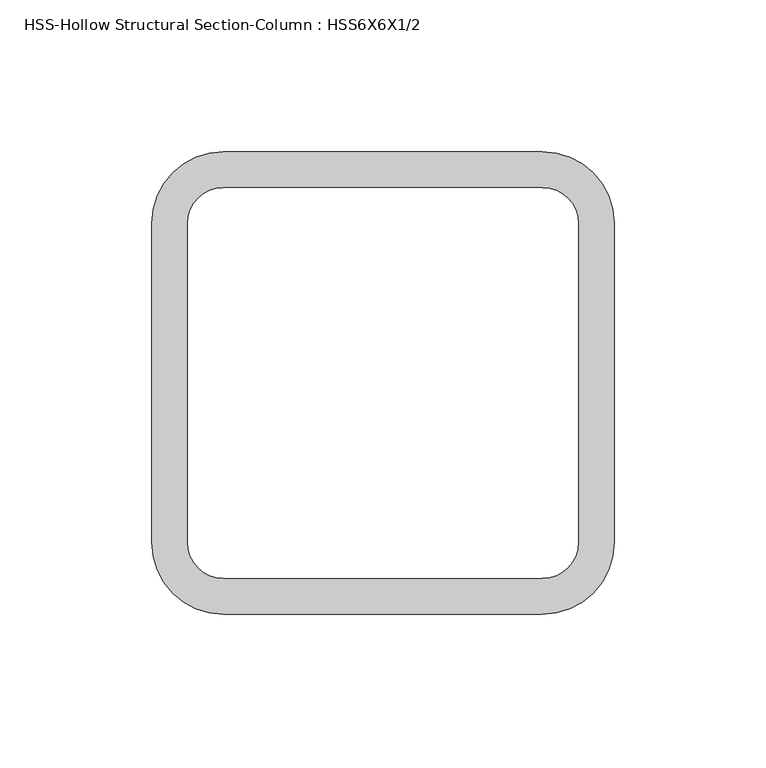
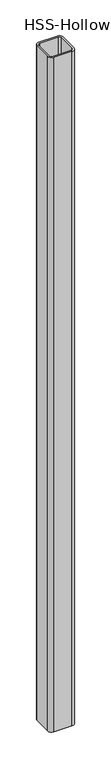
"""IFC4 building model written with IfcOpenShell, lengths in millimetres: column geometry, HSS-Hollow Structural Section-Column : HSS6X6X1/2."""

from ifc_helpers import new_model, si_unit, point, frame_2d, origin, origin_with_axes, place, context, project, spatial, polyline, circle_curve, trimmed, segment, composite_curve, outline, extrude, source, transform, mapped, element, save


def hss_hollow_structural_section_column_hss6x6x1_2_37f7f079(model_context):
    return source(origin(), model_context, "Body", "SweptSolid", [
        extrude(outline(composite_curve([segment(trimmed(circle_curve(frame_2d((52.578, 52.578)), 23.622), [point((52.578, 76.2))], [point((76.2, 52.578))], False, "CARTESIAN"), True, "CONTINUOUS"), segment(polyline([(76.2, 52.578), (76.2, -52.578)]), True, "CONTINUOUS"), segment(trimmed(circle_curve(frame_2d((52.578, -52.578)), 23.622), [point((76.2, -52.578))], [point((52.578, -76.2))], False, "CARTESIAN"), True, "CONTINUOUS"), segment(polyline([(52.578, -76.2), (-52.578, -76.2)]), True, "CONTINUOUS"), segment(trimmed(circle_curve(frame_2d((-52.578, -52.578)), 23.622), [point((-52.578, -76.2))], [point((-76.2, -52.578))], False, "CARTESIAN"), True, "CONTINUOUS"), segment(polyline([(-76.2, -52.578), (-76.2, 52.578)]), True, "CONTINUOUS"), segment(trimmed(circle_curve(frame_2d((-52.578, 52.578)), 23.622), [point((-76.2, 52.578))], [point((-52.578, 76.2))], False, "CARTESIAN"), True, "CONTINUOUS"), segment(polyline([(-52.578, 76.2), (52.578, 76.2)]), True, "CONTINUOUS")], self_intersect=False), holes=[composite_curve([segment(polyline([(52.578, 64.389), (-52.578, 64.389)]), True, "CONTINUOUS"), segment(trimmed(circle_curve(frame_2d((-52.578, 52.578)), 11.811), [point((-52.578, 64.389))], [point((-64.389, 52.578))], True, "CARTESIAN"), True, "CONTINUOUS"), segment(polyline([(-64.389, 52.578), (-64.389, -52.578)]), True, "CONTINUOUS"), segment(trimmed(circle_curve(frame_2d((-52.578, -52.578)), 11.811), [point((-64.389, -52.578))], [point((-52.578, -64.389))], True, "CARTESIAN"), True, "CONTINUOUS"), segment(polyline([(-52.578, -64.389), (52.578, -64.389)]), True, "CONTINUOUS"), segment(trimmed(circle_curve(frame_2d((52.578, -52.578)), 11.811), [point((52.578, -64.389))], [point((64.389, -52.578))], True, "CARTESIAN"), True, "CONTINUOUS"), segment(polyline([(64.389, -52.578), (64.389, 52.578)]), True, "CONTINUOUS"), segment(trimmed(circle_curve(frame_2d((52.578, 52.578)), 11.811), [point((64.389, 52.578))], [point((52.578, 64.389))], True, "CARTESIAN"), True, "CONTINUOUS")], self_intersect=False)]), origin_with_axes(), (0.0, 0.0, 1.0), 4127.5),
    ])


if __name__ == "__main__":
    model = new_model("IFC4")
    model_context = context("Model", 3, world=origin())
    ifc_project = project(units=[si_unit("LENGTHUNIT", "METRE", prefix="MILLI")], contexts=[model_context])
    site = spatial("IfcSite", under=ifc_project)
    building = spatial("IfcBuilding", under=site)
    placement = place(None, origin())
    hss_hollow_structural_section_column_hss6x6x1_2_shape = hss_hollow_structural_section_column_hss6x6x1_2_37f7f079(model_context)
    element("IfcColumn", 1, ObjectType="HSS-Hollow Structural Section-Column : HSS6X6X1/2", at=placement, inside=building, context=model_context, shape_type="MappedRepresentation", body=[
        mapped(hss_hollow_structural_section_column_hss6x6x1_2_shape, transform((0.0, 0.0, 0.0), x_axis=(1.0, 0.0, 0.0), y_axis=(0.0, 1.0, 0.0), z_axis=(0.0, 0.0, 1.0))),
    ])
    save(model, "model.ifc")

# Revit data of these elements
# Type "HSS-Hollow Structural Section-Column : HSS6X6X1/2"
#   Assembly Code = "B10"
#   Shape = "Square"
#   W = 35.1
#   Ht = 0' - 6"
#   b = 0' - 6"
#   kr = 0' - 0.93"
#   t = 0' - 0.465"
#   A = 0.0676389 SF
#   Structural Material [instance default] = Steel ASTM A500, Grade B, Rectangular and Square
# Element 1 (IfcColumn, "HSS-Hollow Structural Section-Column : HSS6X6X1/2")
#   Materials on its faces: "Steel ASTM A500, Grade B, Rectangular and Square"
# Materials
#   "Steel ASTM A500, Grade B, Rectangular and Square": class "Metal", colour RGB 199 199 199, transparency 0, Description = "Carbon steel", Cost = 0
